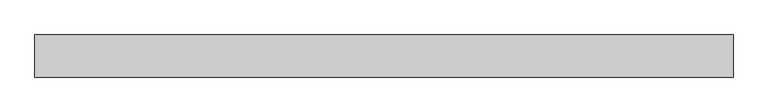
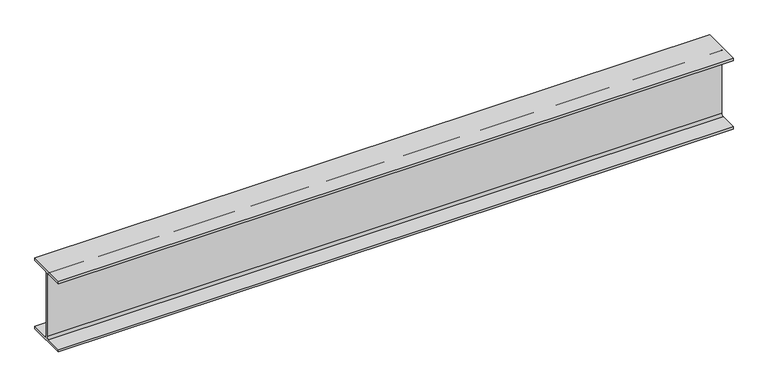
"""IFC4 building model written with IfcOpenShell, lengths in millimetres: beam geometry, Steel Beam_H-KSD3502 : H_SB_ASB_H-200x200x8x12."""

import ifcopenshell
import ifcopenshell.guid

model = None  # the IFC model being written
_history = None  # IfcOwnerHistory: only IFC2X3 demands one
_inside = {}  # id of a spatial element -> (the spatial element, [elements in it])
_under = {}  # id of a project, library or spatial element -> (it, [spatial elements below it])
_declared = {}  # id of a project -> (the project, [libraries it declares])
_typed = {}  # id of a type object -> (the type object, [elements of that type])
_made_of = {}  # id of a material, layer set ... -> (it, [elements and type objects made of it])


def new_model(schema):
    """Start an empty IFC model of exactly this schema.

    Asked for "IFC4X3", IfcOpenShell would pick the latest addendum, in which some entities
    have other attributes; the version numbers below select the first issue.
    IFC2X3 requires an IfcOwnerHistory on every rooted entity: one is made here for all.
    """
    global model, _history
    if schema == "IFC4X3":
        model = ifcopenshell.file(schema_version=(4, 3, 0, 0))
    else:
        model = ifcopenshell.file(schema=schema)
    _inside.clear()
    _under.clear()
    _declared.clear()
    _typed.clear()
    _made_of.clear()
    _history = None
    if model.schema == "IFC2X3":
        org = make("IfcOrganization", Name="unknown")
        user = make(
            "IfcPersonAndOrganization",
            ThePerson=make("IfcPerson", FamilyName="unknown"),
            TheOrganization=org,
        )
        app = make(
            "IfcApplication",
            ApplicationDeveloper=org,
            Version="unknown",
            ApplicationFullName="unknown",
            ApplicationIdentifier="unknown",
        )
        _history = make(
            "IfcOwnerHistory",
            OwningUser=user,
            OwningApplication=app,
            ChangeAction="ADDED",
            CreationDate=0,
        )
    return model


def make(cls, **values):
    """One entity of the class cls with the attributes given. An attribute that is None is left unset."""
    return model.create_entity(
        cls, **{name: value for name, value in values.items() if value is not None}
    )


def rooted(cls, **values):
    """An entity with a GlobalId (a new one), such as an element, a storey or a relation."""
    return make(cls, GlobalId=ifcopenshell.guid.new(), OwnerHistory=_history, **values)


def si_unit(unit_type, name, prefix=None):
    """IfcSIUnit, for example si_unit("LENGTHUNIT", "METRE", prefix="MILLI")."""
    return make("IfcSIUnit", UnitType=unit_type, Prefix=prefix, Name=name)


def assignment(units):
    """IfcUnitAssignment: the units of a project."""
    return None if units is None else make("IfcUnitAssignment", Units=units)


def point(xyz):
    """IfcCartesianPoint."""
    return None if xyz is None else make("IfcCartesianPoint", Coordinates=xyz)


def direction(xyz):
    """IfcDirection."""
    return None if xyz is None else make("IfcDirection", DirectionRatios=xyz)


def frame(location, z_axis=None, x_axis=None):
    """IfcAxis2Placement3D, a coordinate frame: its origin and axes. An axis left out is left unset."""
    return make(
        "IfcAxis2Placement3D",
        Location=point(location),
        Axis=direction(z_axis),
        RefDirection=direction(x_axis),
    )


def frame_2d(location, x_axis=None):
    """IfcAxis2Placement2D, a coordinate frame in the plane: its origin and x axis."""
    return make(
        "IfcAxis2Placement2D", Location=point(location), RefDirection=direction(x_axis)
    )


def origin():
    """The frame at (0, 0, 0) with its axes left unset."""
    return frame((0.0, 0.0, 0.0))


def place(relative_to, where):
    """IfcLocalPlacement: puts the frame where relative to a parent placement (None: the world)."""
    return make(
        "IfcLocalPlacement", PlacementRelTo=relative_to, RelativePlacement=where
    )


def context(
    kind, dimensions, precision=None, world=None, true_north=None, identifier=None
):
    """IfcGeometricRepresentationContext, for example the 3D "Model" context."""
    return make(
        "IfcGeometricRepresentationContext",
        ContextIdentifier=identifier,
        ContextType=kind,
        CoordinateSpaceDimension=dimensions,
        Precision=precision,
        WorldCoordinateSystem=world,
        TrueNorth=true_north,
    )


def project(units=None, contexts=None):
    """IfcProject with its units and contexts."""
    return rooted(
        "IfcProject",
        Name="project",
        RepresentationContexts=contexts,
        UnitsInContext=assignment(units),
    )


def spatial(cls, under=None, at=None, **own):
    """A site, building, storey or space (cls), placed at a placement, below another one or the project."""
    s = rooted(cls, ObjectPlacement=at, **own)
    if under is not None:
        _under.setdefault(under.id(), (under, []))[1].append(s)
    return s


def polyline(points):
    """IfcPolyline through the points."""
    return make("IfcPolyline", Points=[point(p) for p in points])


def circle_curve(where, radius):
    """IfcCircle in the frame where."""
    return make("IfcCircle", Position=where, Radius=radius)


def trimmed(basis, trim1, trim2, sense, master):
    """IfcTrimmedCurve: the piece of a basis curve between two trims."""
    return make(
        "IfcTrimmedCurve",
        BasisCurve=basis,
        Trim1=trim1,
        Trim2=trim2,
        SenseAgreement=sense,
        MasterRepresentation=master,
    )


def segment(curve, same_sense, transition):
    """IfcCompositeCurveSegment."""
    return make(
        "IfcCompositeCurveSegment",
        Transition=transition,
        SameSense=same_sense,
        ParentCurve=curve,
    )


def composite_curve(segments, self_intersect=None):
    """IfcCompositeCurve: segments joined end to end."""
    return make("IfcCompositeCurve", Segments=segments, SelfIntersect=self_intersect)


def outline(outer, holes=None, kind="AREA"):
    """IfcArbitraryClosedProfileDef: a profile drawn as a closed curve; with holes, ...WithVoids."""
    if holes is None:
        return make("IfcArbitraryClosedProfileDef", ProfileType=kind, OuterCurve=outer)
    return make(
        "IfcArbitraryProfileDefWithVoids",
        ProfileType=kind,
        OuterCurve=outer,
        InnerCurves=holes,
    )


def extrude(swept, where, along, depth):
    """IfcExtrudedAreaSolid: the profile swept, set in the frame where, extruded along a direction by depth."""
    return make(
        "IfcExtrudedAreaSolid",
        SweptArea=swept,
        Position=where,
        ExtrudedDirection=direction(along),
        Depth=depth,
    )


def shape(context_of_items, identifier, shape_type, items):
    """IfcShapeRepresentation: the items that make up one representation, for example the "Body"."""
    return make(
        "IfcShapeRepresentation",
        ContextOfItems=context_of_items,
        RepresentationIdentifier=identifier,
        RepresentationType=shape_type,
        Items=items,
    )


def source(mapping_origin, context_of_items, identifier, shape_type, items):
    """IfcRepresentationMap: a shape defined once, which mapped items show again and again."""
    return make(
        "IfcRepresentationMap",
        MappingOrigin=mapping_origin,
        MappedRepresentation=shape(context_of_items, identifier, shape_type, items),
    )


def transform(
    local_origin,
    x_axis=None,
    y_axis=None,
    z_axis=None,
    scale=None,
    scale2=None,
    scale3=None,
    uniform=True,
):
    """IfcCartesianTransformationOperator3D, or its non-uniform kind. x_axis, y_axis, z_axis: its Axis1, 2, 3."""
    if uniform:
        return make(
            "IfcCartesianTransformationOperator3D",
            Axis1=direction(x_axis),
            Axis2=direction(y_axis),
            LocalOrigin=point(local_origin),
            Scale=scale,
            Axis3=direction(z_axis),
        )
    return make(
        "IfcCartesianTransformationOperator3DnonUniform",
        Axis1=direction(x_axis),
        Axis2=direction(y_axis),
        LocalOrigin=point(local_origin),
        Scale=scale,
        Axis3=direction(z_axis),
        Scale2=scale2,
        Scale3=scale3,
    )


def mapped(mapping_source, mapping_target):
    """IfcMappedItem: shows the shape of a source again, moved by a transform."""
    return make(
        "IfcMappedItem", MappingSource=mapping_source, MappingTarget=mapping_target
    )


def made_of(thing, what):
    """Note that an element or type object is made of a material, layer set ...; save() writes the relation."""
    if what is not None:
        _made_of.setdefault(what.id(), (what, []))[1].append(thing)
    return thing


def element(
    cls,
    number,
    at=None,
    inside=None,
    cuts=None,
    type_object=None,
    material=None,
    context=None,
    identifier="Body",
    shape_type=None,
    held_by="IfcProductDefinitionShape",
    body=None,
    shapes=None,
    **own,
):
    """One element of the class cls, such as IfcWall. Its Tag is "e" and its number.

    at: its placement. inside: the storey or other place that contains it. cuts: it is an
    opening in that element (IfcRelVoidsElement). A single representation is given by context,
    identifier, shape_type and body (its items); several are given by shapes. held_by: the class
    of the entity that holds the representations. save() writes the other relations.
    """
    e = rooted(cls, Tag="e%d" % number, ObjectPlacement=at, **own)
    if body is not None:
        shapes = [shape(context, identifier, shape_type, body)]
    if shapes is not None:
        e.Representation = make(held_by, Representations=shapes)
    if inside is not None:
        _inside.setdefault(inside.id(), (inside, []))[1].append(e)
    if cuts is not None:
        rooted(
            "IfcRelVoidsElement", RelatingBuildingElement=cuts, RelatedOpeningElement=e
        )
    if type_object is not None:
        _typed.setdefault(type_object.id(), (type_object, []))[1].append(e)
    return made_of(e, material)


def aggregate(whole, parts):
    """IfcRelAggregates: a whole, such as a stair, and the parts it consists of."""
    return rooted("IfcRelAggregates", RelatingObject=whole, RelatedObjects=parts)


def save(model, path):
    """Write the relations noted so far, then the file.

    IfcRelAggregates (storeys below a building ...), IfcRelContainedInSpatialStructure (elements
    in a storey), IfcRelDefinesByType, IfcRelAssociatesMaterial and IfcRelDeclares: one each for
    every whole, place, type object, material and project.
    """
    for whole, parts in _under.values():
        aggregate(whole, parts)
    for where, things in _inside.values():
        rooted(
            "IfcRelContainedInSpatialStructure",
            RelatedElements=things,
            RelatingStructure=where,
        )
    for kind, things in _typed.values():
        rooted("IfcRelDefinesByType", RelatedObjects=things, RelatingType=kind)
    for what, things in _made_of.values():
        rooted("IfcRelAssociatesMaterial", RelatedObjects=things, RelatingMaterial=what)
    for by, libraries in _declared.values():
        rooted("IfcRelDeclares", RelatingContext=by, RelatedDefinitions=libraries)
    model.write(path)


def beam_0adccc4e(model_context):
    return source(origin(), model_context, "Body", "SweptSolid", [
        extrude(outline(composite_curve([segment(polyline([(82.5, -141.5), (82.5, -151.7), (-82.5, -151.7), (-82.5, -141.5), (-11.9, -141.5)]), True, "CONTINUOUS"), segment(trimmed(circle_curve(frame_2d((-11.9, -132.6)), 8.9), [point((-11.9, -141.5))], [point((-3.0, -132.6))], True, "CARTESIAN"), True, "CONTINUOUS"), segment(polyline([(-3.0, -132.6), (-3.0, 132.6)]), True, "CONTINUOUS"), segment(trimmed(circle_curve(frame_2d((-11.9, 132.6)), 8.9), [point((-3.0, 132.6))], [point((-11.9, 141.5))], True, "CARTESIAN"), True, "CONTINUOUS"), segment(polyline([(-11.9, 141.5), (-82.5, 141.5), (-82.5, 151.7), (82.5, 151.7), (82.5, 141.5), (11.9, 141.5)]), True, "CONTINUOUS"), segment(trimmed(circle_curve(frame_2d((11.9, 132.6)), 8.9), [point((11.9, 141.5))], [point((3.0, 132.6))], True, "CARTESIAN"), True, "CONTINUOUS"), segment(polyline([(3.0, 132.6), (3.0, -132.6)]), True, "CONTINUOUS"), segment(trimmed(circle_curve(frame_2d((11.9, -132.6)), 8.9), [point((3.0, -132.6))], [point((11.9, -141.5))], True, "CARTESIAN"), True, "CONTINUOUS"), segment(polyline([(11.9, -141.5), (82.5, -141.5)]), True, "CONTINUOUS")], self_intersect=False)), frame((-1342.1060823, 0.0, 0.0), z_axis=(1.0, 0.0, 0.0), x_axis=(0.0, 1.0, 0.0)), (0.0, 0.0, 1.0), 2735.8528348),
    ])


if __name__ == "__main__":
    model = new_model("IFC4")
    model_context = context("Model", 3, world=origin())
    ifc_project = project(units=[si_unit("LENGTHUNIT", "METRE", prefix="MILLI")], contexts=[model_context])
    site = spatial("IfcSite", under=ifc_project)
    building = spatial("IfcBuilding", under=site)
    placement = place(None, origin())
    beam_shape = beam_0adccc4e(model_context)
    element("IfcBeam", 1, ObjectType="Steel Beam_H-KSD3502 : H_SB_ASB_H-200x200x8x12", at=placement, inside=building, context=model_context, shape_type="MappedRepresentation", body=[
        mapped(beam_shape, transform((0.0, 0.0, 0.0), x_axis=(1.0, 0.0, 0.0), y_axis=(0.0, 1.0, 0.0), z_axis=(0.0, 0.0, 1.0))),
    ])
    save(model, "model.ifc")

# Revit data of these elements
# Type "Steel Beam_H-KSD3502 : H_SB_ASB_H-200x200x8x12"
#   Width = 20.0 cm
#   Web Thickness = 0.8 cm
#   Web Fillet = 1.3 cm
#   Warping Constant = 141376.0 cm⁶
#   Torsional Moment of Inertia = 26.2485 cm⁴
#   Torsional Modulus = 1.0 cm³
#   Section Area = 63.53 cm²
#   Plastic Modulus weak axis = 244.0 cm³
#   Plastic Modulus strong axis = 525.0 cm³
#   Perimeter = 1.16 m²/m
#   Nominal Weight = 49.90 kgf/m
#   Moment of Inertia weak axis = 1600.00 cm⁴
#   Moment of Inertia strong axis = 4720.00 cm⁴
#   Height = 20.0 cm
#   Flange Thickness = 1.2 cm
#   Elastic Modulus weak axis = 160.0 cm³
#   Elastic Modulus strong axis = 472.0 cm³
#   Centroid Vertical = 10.0 cm
#   Centroid Horizontal = 10.0 cm
#   Length [instance default] = 1.5240 m
#   Structural Material [instance default] = Steel, 45-345
#   Assembly Code = ""
# Element 1 (IfcBeam, "Steel Beam_H-KSD3502 : H_SB_ASB_H-200x200x8x12")
#   Structural Material = none
# Materials
#   "Steel, 45-345": class "Metal", colour RGB 189 187 185, transparency 0, Description = "Steel 345 MPa", Cost = 0
